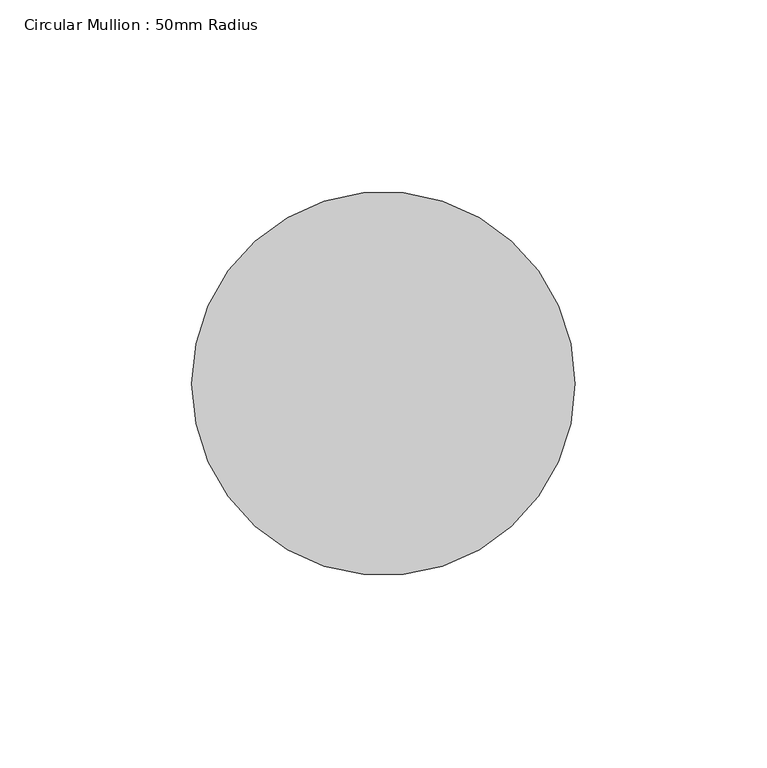
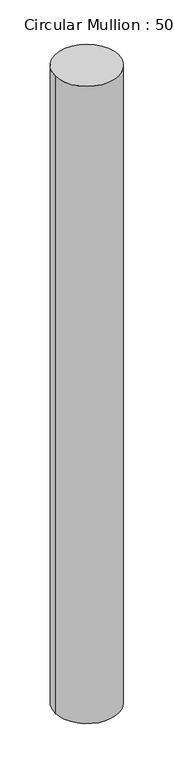
"""IFC4 building model written with IfcOpenShell, lengths in millimetres: member geometry, Circular Mullion : 50mm Radius."""

from ifc_helpers import new_model, si_unit, point, frame, origin, origin_2d, place, context, project, spatial, circle_curve, trimmed, segment, composite_curve, outline, extrude, source, transform, mapped, element, save


def circular_mullion_50mm_radius_3c5d97c9(model_context):
    return source(origin(), model_context, "Body", "SweptSolid", [
        extrude(outline(composite_curve([segment(trimmed(circle_curve(origin_2d(), 50.0), [point((50.0, 0.0))], [point((-50.0, 0.0))], False, "CARTESIAN"), True, "CONTINUOUS"), segment(trimmed(circle_curve(origin_2d(), 50.0), [point((-50.0, 0.0))], [point((50.0, 0.0))], False, "CARTESIAN"), True, "CONTINUOUS")], self_intersect=False)), frame((0.0, 0.0, -1060.7501868), z_axis=(0.0, 0.0, 1.0), x_axis=(1.0, 0.0, 0.0)), (0.0, 0.0, 1.0), 1060.7501868),
    ])


if __name__ == "__main__":
    model = new_model("IFC4")
    model_context = context("Model", 3, world=origin())
    ifc_project = project(units=[si_unit("LENGTHUNIT", "METRE", prefix="MILLI")], contexts=[model_context])
    site = spatial("IfcSite", under=ifc_project)
    building = spatial("IfcBuilding", under=site)
    placement = place(None, origin())
    circular_mullion_50mm_radius_shape = circular_mullion_50mm_radius_3c5d97c9(model_context)
    element("IfcMember", 1, ObjectType="Circular Mullion : 50mm Radius", at=placement, inside=building, context=model_context, shape_type="MappedRepresentation", body=[
        mapped(circular_mullion_50mm_radius_shape, transform((0.0, 0.0, 0.0), x_axis=(1.0, 0.0, 0.0), y_axis=(0.0, 1.0, 0.0), z_axis=(0.0, 0.0, 1.0))),
    ])
    save(model, "model.ifc")

# Revit data of these elements
# Type "Circular Mullion : 50mm Radius"
#   built-in parameter 1007350 = 0.164042 (stored number, unit not read)
# Element 1 (IfcMember, "Circular Mullion : 50mm Radius")
#   Materials on its faces: "Aluminium"
# Materials
#   "Aluminium": class "Metal", colour RGB 247 247 247, transparency 0, Description = "Aluminium 6061", Cost = 0
